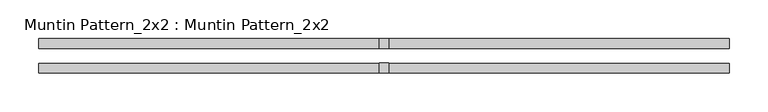
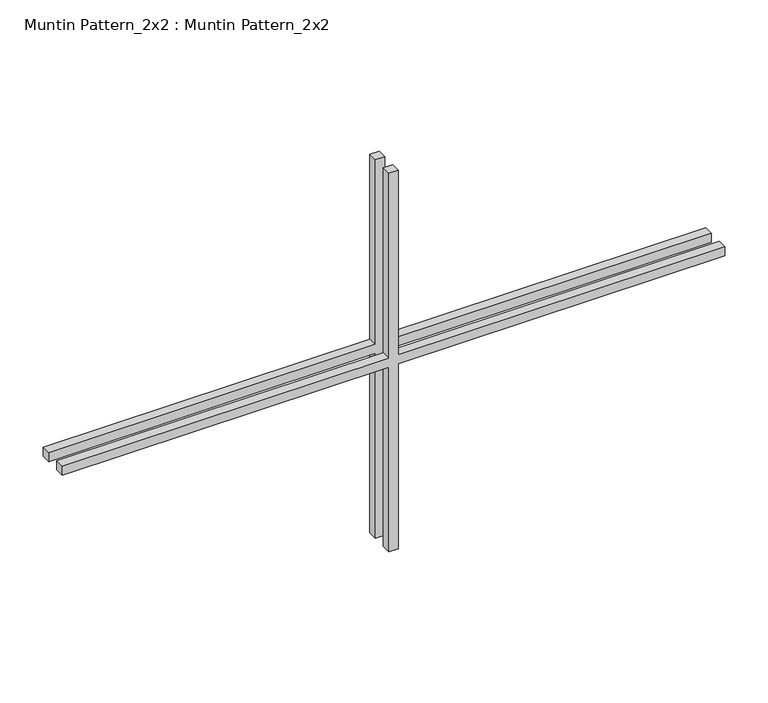
"""IFC4 building model written with IfcOpenShell, lengths in millimetres: proxy geometry, Muntin Pattern_2x2 : Muntin Pattern_2x2."""

import ifcopenshell
import ifcopenshell.guid

model = None  # the IFC model being written
_history = None  # IfcOwnerHistory: only IFC2X3 demands one
_inside = {}  # id of a spatial element -> (the spatial element, [elements in it])
_under = {}  # id of a project, library or spatial element -> (it, [spatial elements below it])
_declared = {}  # id of a project -> (the project, [libraries it declares])
_typed = {}  # id of a type object -> (the type object, [elements of that type])
_made_of = {}  # id of a material, layer set ... -> (it, [elements and type objects made of it])


def new_model(schema):
    """Start an empty IFC model of exactly this schema.

    Asked for "IFC4X3", IfcOpenShell would pick the latest addendum, in which some entities
    have other attributes; the version numbers below select the first issue.
    IFC2X3 requires an IfcOwnerHistory on every rooted entity: one is made here for all.
    """
    global model, _history
    if schema == "IFC4X3":
        model = ifcopenshell.file(schema_version=(4, 3, 0, 0))
    else:
        model = ifcopenshell.file(schema=schema)
    _inside.clear()
    _under.clear()
    _declared.clear()
    _typed.clear()
    _made_of.clear()
    _history = None
    if model.schema == "IFC2X3":
        org = make("IfcOrganization", Name="unknown")
        user = make(
            "IfcPersonAndOrganization",
            ThePerson=make("IfcPerson", FamilyName="unknown"),
            TheOrganization=org,
        )
        app = make(
            "IfcApplication",
            ApplicationDeveloper=org,
            Version="unknown",
            ApplicationFullName="unknown",
            ApplicationIdentifier="unknown",
        )
        _history = make(
            "IfcOwnerHistory",
            OwningUser=user,
            OwningApplication=app,
            ChangeAction="ADDED",
            CreationDate=0,
        )
    return model


def make(cls, **values):
    """One entity of the class cls with the attributes given. An attribute that is None is left unset."""
    return model.create_entity(
        cls, **{name: value for name, value in values.items() if value is not None}
    )


def rooted(cls, **values):
    """An entity with a GlobalId (a new one), such as an element, a storey or a relation."""
    return make(cls, GlobalId=ifcopenshell.guid.new(), OwnerHistory=_history, **values)


def si_unit(unit_type, name, prefix=None):
    """IfcSIUnit, for example si_unit("LENGTHUNIT", "METRE", prefix="MILLI")."""
    return make("IfcSIUnit", UnitType=unit_type, Prefix=prefix, Name=name)


def assignment(units):
    """IfcUnitAssignment: the units of a project."""
    return None if units is None else make("IfcUnitAssignment", Units=units)


def point(xyz):
    """IfcCartesianPoint."""
    return None if xyz is None else make("IfcCartesianPoint", Coordinates=xyz)


def direction(xyz):
    """IfcDirection."""
    return None if xyz is None else make("IfcDirection", DirectionRatios=xyz)


def frame(location, z_axis=None, x_axis=None):
    """IfcAxis2Placement3D, a coordinate frame: its origin and axes. An axis left out is left unset."""
    return make(
        "IfcAxis2Placement3D",
        Location=point(location),
        Axis=direction(z_axis),
        RefDirection=direction(x_axis),
    )


def origin():
    """The frame at (0, 0, 0) with its axes left unset."""
    return frame((0.0, 0.0, 0.0))


def place(relative_to, where):
    """IfcLocalPlacement: puts the frame where relative to a parent placement (None: the world)."""
    return make(
        "IfcLocalPlacement", PlacementRelTo=relative_to, RelativePlacement=where
    )


def context(
    kind, dimensions, precision=None, world=None, true_north=None, identifier=None
):
    """IfcGeometricRepresentationContext, for example the 3D "Model" context."""
    return make(
        "IfcGeometricRepresentationContext",
        ContextIdentifier=identifier,
        ContextType=kind,
        CoordinateSpaceDimension=dimensions,
        Precision=precision,
        WorldCoordinateSystem=world,
        TrueNorth=true_north,
    )


def project(units=None, contexts=None):
    """IfcProject with its units and contexts."""
    return rooted(
        "IfcProject",
        Name="project",
        RepresentationContexts=contexts,
        UnitsInContext=assignment(units),
    )


def spatial(cls, under=None, at=None, **own):
    """A site, building, storey or space (cls), placed at a placement, below another one or the project."""
    s = rooted(cls, ObjectPlacement=at, **own)
    if under is not None:
        _under.setdefault(under.id(), (under, []))[1].append(s)
    return s


def polyline(points):
    """IfcPolyline through the points."""
    return make("IfcPolyline", Points=[point(p) for p in points])


def outline(outer, holes=None, kind="AREA"):
    """IfcArbitraryClosedProfileDef: a profile drawn as a closed curve; with holes, ...WithVoids."""
    if holes is None:
        return make("IfcArbitraryClosedProfileDef", ProfileType=kind, OuterCurve=outer)
    return make(
        "IfcArbitraryProfileDefWithVoids",
        ProfileType=kind,
        OuterCurve=outer,
        InnerCurves=holes,
    )


def extrude(swept, where, along, depth):
    """IfcExtrudedAreaSolid: the profile swept, set in the frame where, extruded along a direction by depth."""
    return make(
        "IfcExtrudedAreaSolid",
        SweptArea=swept,
        Position=where,
        ExtrudedDirection=direction(along),
        Depth=depth,
    )


def shape(context_of_items, identifier, shape_type, items):
    """IfcShapeRepresentation: the items that make up one representation, for example the "Body"."""
    return make(
        "IfcShapeRepresentation",
        ContextOfItems=context_of_items,
        RepresentationIdentifier=identifier,
        RepresentationType=shape_type,
        Items=items,
    )


def source(mapping_origin, context_of_items, identifier, shape_type, items):
    """IfcRepresentationMap: a shape defined once, which mapped items show again and again."""
    return make(
        "IfcRepresentationMap",
        MappingOrigin=mapping_origin,
        MappedRepresentation=shape(context_of_items, identifier, shape_type, items),
    )


def transform(
    local_origin,
    x_axis=None,
    y_axis=None,
    z_axis=None,
    scale=None,
    scale2=None,
    scale3=None,
    uniform=True,
):
    """IfcCartesianTransformationOperator3D, or its non-uniform kind. x_axis, y_axis, z_axis: its Axis1, 2, 3."""
    if uniform:
        return make(
            "IfcCartesianTransformationOperator3D",
            Axis1=direction(x_axis),
            Axis2=direction(y_axis),
            LocalOrigin=point(local_origin),
            Scale=scale,
            Axis3=direction(z_axis),
        )
    return make(
        "IfcCartesianTransformationOperator3DnonUniform",
        Axis1=direction(x_axis),
        Axis2=direction(y_axis),
        LocalOrigin=point(local_origin),
        Scale=scale,
        Axis3=direction(z_axis),
        Scale2=scale2,
        Scale3=scale3,
    )


def mapped(mapping_source, mapping_target):
    """IfcMappedItem: shows the shape of a source again, moved by a transform."""
    return make(
        "IfcMappedItem", MappingSource=mapping_source, MappingTarget=mapping_target
    )


def made_of(thing, what):
    """Note that an element or type object is made of a material, layer set ...; save() writes the relation."""
    if what is not None:
        _made_of.setdefault(what.id(), (what, []))[1].append(thing)
    return thing


def element(
    cls,
    number,
    at=None,
    inside=None,
    cuts=None,
    type_object=None,
    material=None,
    context=None,
    identifier="Body",
    shape_type=None,
    held_by="IfcProductDefinitionShape",
    body=None,
    shapes=None,
    **own,
):
    """One element of the class cls, such as IfcWall. Its Tag is "e" and its number.

    at: its placement. inside: the storey or other place that contains it. cuts: it is an
    opening in that element (IfcRelVoidsElement). A single representation is given by context,
    identifier, shape_type and body (its items); several are given by shapes. held_by: the class
    of the entity that holds the representations. save() writes the other relations.
    """
    e = rooted(cls, Tag="e%d" % number, ObjectPlacement=at, **own)
    if body is not None:
        shapes = [shape(context, identifier, shape_type, body)]
    if shapes is not None:
        e.Representation = make(held_by, Representations=shapes)
    if inside is not None:
        _inside.setdefault(inside.id(), (inside, []))[1].append(e)
    if cuts is not None:
        rooted(
            "IfcRelVoidsElement", RelatingBuildingElement=cuts, RelatedOpeningElement=e
        )
    if type_object is not None:
        _typed.setdefault(type_object.id(), (type_object, []))[1].append(e)
    return made_of(e, material)


def aggregate(whole, parts):
    """IfcRelAggregates: a whole, such as a stair, and the parts it consists of."""
    return rooted("IfcRelAggregates", RelatingObject=whole, RelatedObjects=parts)


def save(model, path):
    """Write the relations noted so far, then the file.

    IfcRelAggregates (storeys below a building ...), IfcRelContainedInSpatialStructure (elements
    in a storey), IfcRelDefinesByType, IfcRelAssociatesMaterial and IfcRelDeclares: one each for
    every whole, place, type object, material and project.
    """
    for whole, parts in _under.values():
        aggregate(whole, parts)
    for where, things in _inside.values():
        rooted(
            "IfcRelContainedInSpatialStructure",
            RelatedElements=things,
            RelatingStructure=where,
        )
    for kind, things in _typed.values():
        rooted("IfcRelDefinesByType", RelatedObjects=things, RelatingType=kind)
    for what, things in _made_of.values():
        rooted("IfcRelAssociatesMaterial", RelatedObjects=things, RelatingMaterial=what)
    for by, libraries in _declared.values():
        rooted("IfcRelDeclares", RelatingContext=by, RelatedDefinitions=libraries)
    model.write(path)


def muntin_pattern_2x2_muntin_pattern_2x2_e5078fa2(model_context):
    return source(origin(), model_context, "Body", "SweptSolid", [
        extrude(outline(polyline([(274.6375, -6.35), (274.6375, -444.5), (261.9375, -444.5), (261.9375, -6.35), (0.0, -6.35), (0.0, 6.35), (261.9375, 6.35), (261.9375, 444.5), (274.6375, 444.5), (274.6375, 6.35), (536.575, 6.35), (536.575, -6.35), (274.6375, -6.35)])), frame((0.0, 9.525, 0.0), z_axis=(0.0, 1.0, 0.0), x_axis=(0.0, 0.0, 1.0)), (0.0, 0.0, 1.0), 12.7),
        extrude(outline(polyline([(274.6375, -6.35), (274.6375, -444.5), (261.9375, -444.5), (261.9375, -6.35), (0.0, -6.35), (0.0, 6.35), (261.9375, 6.35), (261.9375, 444.5), (274.6375, 444.5), (274.6375, 6.35), (536.575, 6.35), (536.575, -6.35), (274.6375, -6.35)])), frame((0.0, -22.225, 0.0), z_axis=(0.0, 1.0, 0.0), x_axis=(0.0, 0.0, 1.0)), (0.0, 0.0, 1.0), 12.7),
    ])


if __name__ == "__main__":
    model = new_model("IFC4")
    model_context = context("Model", 3, world=origin())
    ifc_project = project(units=[si_unit("LENGTHUNIT", "METRE", prefix="MILLI")], contexts=[model_context])
    site = spatial("IfcSite", under=ifc_project)
    building = spatial("IfcBuilding", under=site)
    placement = place(None, origin())
    muntin_pattern_2x2_muntin_pattern_2x2_shape = muntin_pattern_2x2_muntin_pattern_2x2_e5078fa2(model_context)
    element("IfcBuildingElementProxy", 1, Name="Muntin Pattern_2x2 : Muntin Pattern_2x2", ObjectType="Muntin Pattern_2x2 : Muntin Pattern_2x2", at=placement, inside=building, context=model_context, shape_type="MappedRepresentation", body=[
        mapped(muntin_pattern_2x2_muntin_pattern_2x2_shape, transform((0.0, 0.0, 0.0), x_axis=(1.0, 0.0, 0.0), y_axis=(0.0, 1.0, 0.0), z_axis=(0.0, 0.0, 1.0))),
    ])
    save(model, "model.ifc")

# Revit data of these elements
# Type "Muntin Pattern_2x2 : Muntin Pattern_2x2"
#   Width [instance default] = 4' - 0"
#   Thickness = 0' - 0 1/2"
#   Height [instance default] = 4' - 0"
#   Distance = 0' - 0 3/4"
#   Interior Material [instance default] = none
#   Exterior Material [instance default] = none
# Element 1 (IfcBuildingElementProxy, "Muntin Pattern_2x2 : Muntin Pattern_2x2")
#   Width = 2' - 11"
#   Height = 1' - 9 1/8"
#   Interior Material = Wood - Stained
#   Exterior Material = Clad - White
#   Materials on its faces: "Clad - White", "Wood - Stained"
# Materials
#   "Clad - White": class "Wood", colour RGB 242 242 238, transparency 0, Cost = 0
#   "Wood - Stained": class "Wood", colour RGB 224 178 126, transparency 0, Cost = 0
